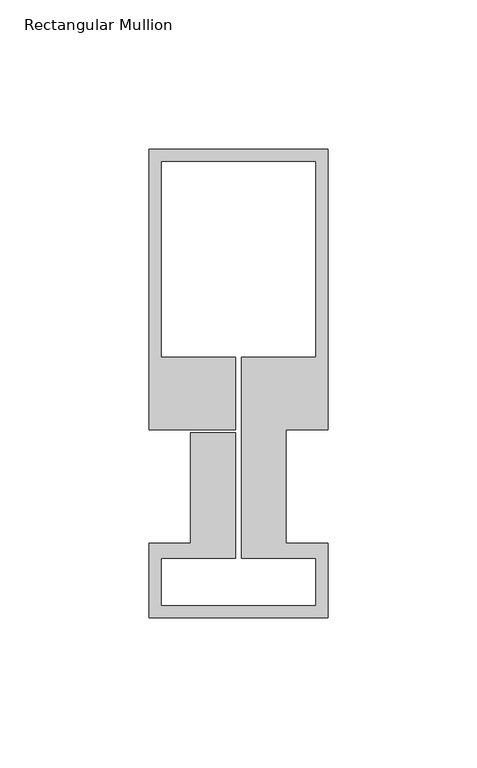
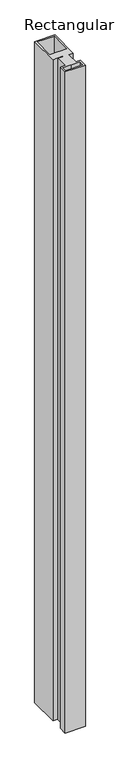
"""IFC4 building model written with IfcOpenShell, lengths in millimetres: member geometry, Rectangular Mullion : Schueco_FWS-60-SI_Mull_CovCap-20mm_Mull-85mm."""

from ifc_helpers import new_model, si_unit, frame, origin, place, context, project, spatial, polyline, outline, extrude, source, transform, mapped, element, save


def rectangular_mullion_b104e485(model_context):
    return source(origin(), model_context, "Body", "SweptSolid", [
        extrude(outline(polyline([(0.0, 132.0), (0.0, 38.0), (-14.0, 38.0), (-14.0, -0.1), (0.0, -0.1), (0.0, -25.0), (-60.0, -25.0), (-60.0, -0.1), (-46.0, -0.1), (-46.0, 37.0), (-31.0, 37.0), (-31.0, -5.0), (-56.0, -5.0), (-56.0, -21.0), (-4.0, -21.0), (-4.0, -5.0), (-29.0, -5.0), (-29.0, 62.3), (-4.0, 62.3), (-4.0, 128.0), (-56.0, 128.0), (-56.0, 62.3), (-31.0, 62.3), (-31.0, 38.0), (-60.0, 38.0), (-60.0, 132.0), (0.0, 132.0)])), frame((0.0, 0.0, -2080.0), z_axis=(0.0, 0.0, 1.0), x_axis=(1.0, 0.0, 0.0)), (0.0, 0.0, 1.0), 2080.0),
    ])


if __name__ == "__main__":
    model = new_model("IFC4")
    model_context = context("Model", 3, world=origin())
    ifc_project = project(units=[si_unit("LENGTHUNIT", "METRE", prefix="MILLI")], contexts=[model_context])
    site = spatial("IfcSite", under=ifc_project)
    building = spatial("IfcBuilding", under=site)
    placement = place(None, origin())
    rectangular_mullion_shape = rectangular_mullion_b104e485(model_context)
    element("IfcMember", 1, ObjectType="Rectangular Mullion : Schueco_FWS-60-SI_Mull_CovCap-20mm_Mull-85mm", at=placement, inside=building, context=model_context, shape_type="MappedRepresentation", body=[
        mapped(rectangular_mullion_shape, transform((0.0, 0.0, 0.0), x_axis=(1.0, 0.0, 0.0), y_axis=(0.0, 1.0, 0.0), z_axis=(0.0, 0.0, 1.0))),
    ])
    save(model, "model.ifc")

# Revit data of these elements
# Type "Rectangular Mullion : Schueco_FWS-60-SI_Mull_CovCap-20mm_Mull-85mm"
#   Model = "FWS 60.SI"
#   Manufacturer = "Schueco International KG"
#   Type Comments = "Mullion"
#   Schueco thermal insulation standard = "Suitable for passive houses"
#   Burglar resistance = "RC 3"
#   Thermal insulation = "to 0.70 W/(m²K)"
#   built-in parameter 1007322 = 0.515092 (stored number, unit not read)
#   built-in parameter 1007321 = 0.0524934 (stored number, unit not read)
#   built-in parameter 1007320 = 0.0524934 (stored number, unit not read)
# Element 1 (IfcMember, "Rectangular Mullion : Schueco_FWS-60-SI_Mull_CovCap-20mm_Mull-85mm")
#   Materials on its faces: "Alu"
# Materials
#   "Alu": class "Glas", colour RGB 140 140 140, transparency 0
